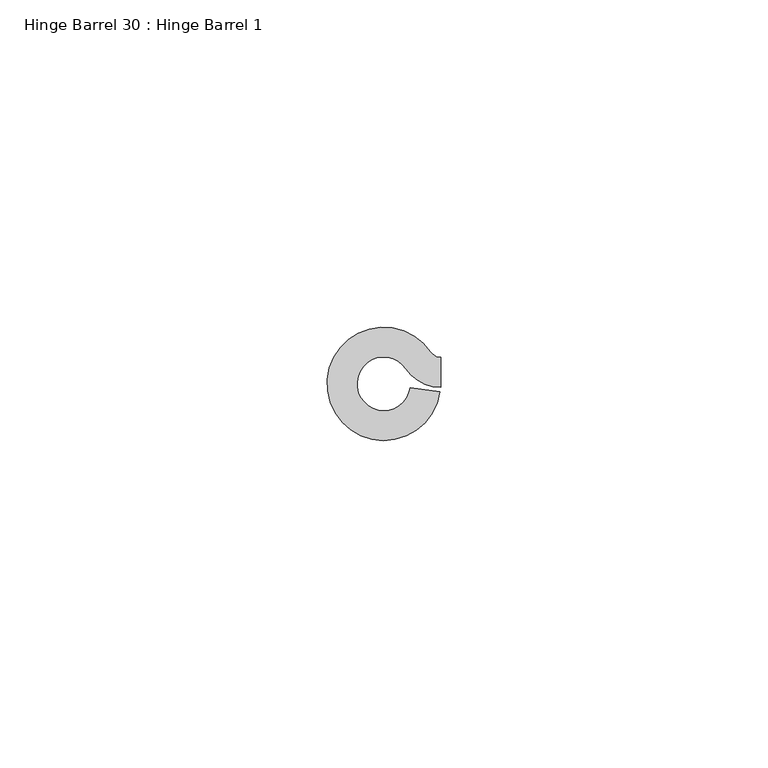
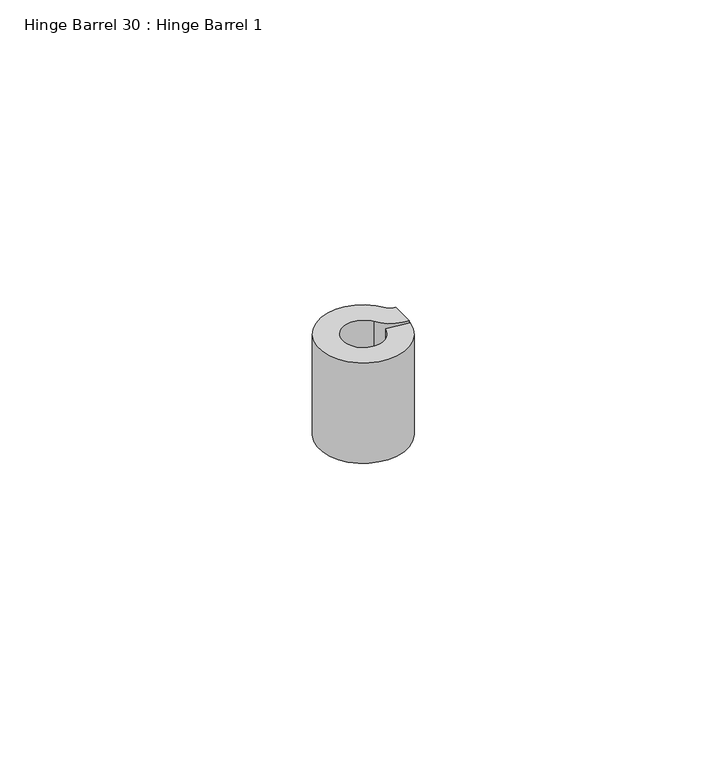
"""IFC4 building model written with IfcOpenShell, lengths in millimetres: proxy geometry, Hinge Barrel 30 : Hinge Barrel 1."""

import ifcopenshell
import ifcopenshell.guid

model = None  # the IFC model being written
_history = None  # IfcOwnerHistory: only IFC2X3 demands one
_inside = {}  # id of a spatial element -> (the spatial element, [elements in it])
_under = {}  # id of a project, library or spatial element -> (it, [spatial elements below it])
_declared = {}  # id of a project -> (the project, [libraries it declares])
_typed = {}  # id of a type object -> (the type object, [elements of that type])
_made_of = {}  # id of a material, layer set ... -> (it, [elements and type objects made of it])


def new_model(schema):
    """Start an empty IFC model of exactly this schema.

    Asked for "IFC4X3", IfcOpenShell would pick the latest addendum, in which some entities
    have other attributes; the version numbers below select the first issue.
    IFC2X3 requires an IfcOwnerHistory on every rooted entity: one is made here for all.
    """
    global model, _history
    if schema == "IFC4X3":
        model = ifcopenshell.file(schema_version=(4, 3, 0, 0))
    else:
        model = ifcopenshell.file(schema=schema)
    _inside.clear()
    _under.clear()
    _declared.clear()
    _typed.clear()
    _made_of.clear()
    _history = None
    if model.schema == "IFC2X3":
        org = make("IfcOrganization", Name="unknown")
        user = make(
            "IfcPersonAndOrganization",
            ThePerson=make("IfcPerson", FamilyName="unknown"),
            TheOrganization=org,
        )
        app = make(
            "IfcApplication",
            ApplicationDeveloper=org,
            Version="unknown",
            ApplicationFullName="unknown",
            ApplicationIdentifier="unknown",
        )
        _history = make(
            "IfcOwnerHistory",
            OwningUser=user,
            OwningApplication=app,
            ChangeAction="ADDED",
            CreationDate=0,
        )
    return model


def make(cls, **values):
    """One entity of the class cls with the attributes given. An attribute that is None is left unset."""
    return model.create_entity(
        cls, **{name: value for name, value in values.items() if value is not None}
    )


def rooted(cls, **values):
    """An entity with a GlobalId (a new one), such as an element, a storey or a relation."""
    return make(cls, GlobalId=ifcopenshell.guid.new(), OwnerHistory=_history, **values)


def si_unit(unit_type, name, prefix=None):
    """IfcSIUnit, for example si_unit("LENGTHUNIT", "METRE", prefix="MILLI")."""
    return make("IfcSIUnit", UnitType=unit_type, Prefix=prefix, Name=name)


def assignment(units):
    """IfcUnitAssignment: the units of a project."""
    return None if units is None else make("IfcUnitAssignment", Units=units)


def point(xyz):
    """IfcCartesianPoint."""
    return None if xyz is None else make("IfcCartesianPoint", Coordinates=xyz)


def direction(xyz):
    """IfcDirection."""
    return None if xyz is None else make("IfcDirection", DirectionRatios=xyz)


def frame(location, z_axis=None, x_axis=None):
    """IfcAxis2Placement3D, a coordinate frame: its origin and axes. An axis left out is left unset."""
    return make(
        "IfcAxis2Placement3D",
        Location=point(location),
        Axis=direction(z_axis),
        RefDirection=direction(x_axis),
    )


def frame_2d(location, x_axis=None):
    """IfcAxis2Placement2D, a coordinate frame in the plane: its origin and x axis."""
    return make(
        "IfcAxis2Placement2D", Location=point(location), RefDirection=direction(x_axis)
    )


def origin():
    """The frame at (0, 0, 0) with its axes left unset."""
    return frame((0.0, 0.0, 0.0))


def place(relative_to, where):
    """IfcLocalPlacement: puts the frame where relative to a parent placement (None: the world)."""
    return make(
        "IfcLocalPlacement", PlacementRelTo=relative_to, RelativePlacement=where
    )


def context(
    kind, dimensions, precision=None, world=None, true_north=None, identifier=None
):
    """IfcGeometricRepresentationContext, for example the 3D "Model" context."""
    return make(
        "IfcGeometricRepresentationContext",
        ContextIdentifier=identifier,
        ContextType=kind,
        CoordinateSpaceDimension=dimensions,
        Precision=precision,
        WorldCoordinateSystem=world,
        TrueNorth=true_north,
    )


def project(units=None, contexts=None):
    """IfcProject with its units and contexts."""
    return rooted(
        "IfcProject",
        Name="project",
        RepresentationContexts=contexts,
        UnitsInContext=assignment(units),
    )


def spatial(cls, under=None, at=None, **own):
    """A site, building, storey or space (cls), placed at a placement, below another one or the project."""
    s = rooted(cls, ObjectPlacement=at, **own)
    if under is not None:
        _under.setdefault(under.id(), (under, []))[1].append(s)
    return s


def polyline(points):
    """IfcPolyline through the points."""
    return make("IfcPolyline", Points=[point(p) for p in points])


def circle_curve(where, radius):
    """IfcCircle in the frame where."""
    return make("IfcCircle", Position=where, Radius=radius)


def trimmed(basis, trim1, trim2, sense, master):
    """IfcTrimmedCurve: the piece of a basis curve between two trims."""
    return make(
        "IfcTrimmedCurve",
        BasisCurve=basis,
        Trim1=trim1,
        Trim2=trim2,
        SenseAgreement=sense,
        MasterRepresentation=master,
    )


def segment(curve, same_sense, transition):
    """IfcCompositeCurveSegment."""
    return make(
        "IfcCompositeCurveSegment",
        Transition=transition,
        SameSense=same_sense,
        ParentCurve=curve,
    )


def composite_curve(segments, self_intersect=None):
    """IfcCompositeCurve: segments joined end to end."""
    return make("IfcCompositeCurve", Segments=segments, SelfIntersect=self_intersect)


def outline(outer, holes=None, kind="AREA"):
    """IfcArbitraryClosedProfileDef: a profile drawn as a closed curve; with holes, ...WithVoids."""
    if holes is None:
        return make("IfcArbitraryClosedProfileDef", ProfileType=kind, OuterCurve=outer)
    return make(
        "IfcArbitraryProfileDefWithVoids",
        ProfileType=kind,
        OuterCurve=outer,
        InnerCurves=holes,
    )


def extrude(swept, where, along, depth):
    """IfcExtrudedAreaSolid: the profile swept, set in the frame where, extruded along a direction by depth."""
    return make(
        "IfcExtrudedAreaSolid",
        SweptArea=swept,
        Position=where,
        ExtrudedDirection=direction(along),
        Depth=depth,
    )


def shape(context_of_items, identifier, shape_type, items):
    """IfcShapeRepresentation: the items that make up one representation, for example the "Body"."""
    return make(
        "IfcShapeRepresentation",
        ContextOfItems=context_of_items,
        RepresentationIdentifier=identifier,
        RepresentationType=shape_type,
        Items=items,
    )


def source(mapping_origin, context_of_items, identifier, shape_type, items):
    """IfcRepresentationMap: a shape defined once, which mapped items show again and again."""
    return make(
        "IfcRepresentationMap",
        MappingOrigin=mapping_origin,
        MappedRepresentation=shape(context_of_items, identifier, shape_type, items),
    )


def transform(
    local_origin,
    x_axis=None,
    y_axis=None,
    z_axis=None,
    scale=None,
    scale2=None,
    scale3=None,
    uniform=True,
):
    """IfcCartesianTransformationOperator3D, or its non-uniform kind. x_axis, y_axis, z_axis: its Axis1, 2, 3."""
    if uniform:
        return make(
            "IfcCartesianTransformationOperator3D",
            Axis1=direction(x_axis),
            Axis2=direction(y_axis),
            LocalOrigin=point(local_origin),
            Scale=scale,
            Axis3=direction(z_axis),
        )
    return make(
        "IfcCartesianTransformationOperator3DnonUniform",
        Axis1=direction(x_axis),
        Axis2=direction(y_axis),
        LocalOrigin=point(local_origin),
        Scale=scale,
        Axis3=direction(z_axis),
        Scale2=scale2,
        Scale3=scale3,
    )


def mapped(mapping_source, mapping_target):
    """IfcMappedItem: shows the shape of a source again, moved by a transform."""
    return make(
        "IfcMappedItem", MappingSource=mapping_source, MappingTarget=mapping_target
    )


def made_of(thing, what):
    """Note that an element or type object is made of a material, layer set ...; save() writes the relation."""
    if what is not None:
        _made_of.setdefault(what.id(), (what, []))[1].append(thing)
    return thing


def element(
    cls,
    number,
    at=None,
    inside=None,
    cuts=None,
    type_object=None,
    material=None,
    context=None,
    identifier="Body",
    shape_type=None,
    held_by="IfcProductDefinitionShape",
    body=None,
    shapes=None,
    **own,
):
    """One element of the class cls, such as IfcWall. Its Tag is "e" and its number.

    at: its placement. inside: the storey or other place that contains it. cuts: it is an
    opening in that element (IfcRelVoidsElement). A single representation is given by context,
    identifier, shape_type and body (its items); several are given by shapes. held_by: the class
    of the entity that holds the representations. save() writes the other relations.
    """
    e = rooted(cls, Tag="e%d" % number, ObjectPlacement=at, **own)
    if body is not None:
        shapes = [shape(context, identifier, shape_type, body)]
    if shapes is not None:
        e.Representation = make(held_by, Representations=shapes)
    if inside is not None:
        _inside.setdefault(inside.id(), (inside, []))[1].append(e)
    if cuts is not None:
        rooted(
            "IfcRelVoidsElement", RelatingBuildingElement=cuts, RelatedOpeningElement=e
        )
    if type_object is not None:
        _typed.setdefault(type_object.id(), (type_object, []))[1].append(e)
    return made_of(e, material)


def aggregate(whole, parts):
    """IfcRelAggregates: a whole, such as a stair, and the parts it consists of."""
    return rooted("IfcRelAggregates", RelatingObject=whole, RelatedObjects=parts)


def save(model, path):
    """Write the relations noted so far, then the file.

    IfcRelAggregates (storeys below a building ...), IfcRelContainedInSpatialStructure (elements
    in a storey), IfcRelDefinesByType, IfcRelAssociatesMaterial and IfcRelDeclares: one each for
    every whole, place, type object, material and project.
    """
    for whole, parts in _under.values():
        aggregate(whole, parts)
    for where, things in _inside.values():
        rooted(
            "IfcRelContainedInSpatialStructure",
            RelatedElements=things,
            RelatingStructure=where,
        )
    for kind, things in _typed.values():
        rooted("IfcRelDefinesByType", RelatedObjects=things, RelatingType=kind)
    for what, things in _made_of.values():
        rooted("IfcRelAssociatesMaterial", RelatedObjects=things, RelatingMaterial=what)
    for by, libraries in _declared.values():
        rooted("IfcRelDeclares", RelatingContext=by, RelatedDefinitions=libraries)
    model.write(path)


def hinge_barrel_30_hinge_barrel_1_18e6ea9c(model_context):
    return source(origin(), model_context, "Body", "SweptSolid", [
        extrude(outline(composite_curve([segment(trimmed(circle_curve(frame_2d((587319.1320739, -531776.6049841)), 4.0894), [point((587322.5194669, -531774.3139665))], [point((587323.1821338, -531777.1708529))], True, "CARTESIAN"), True, "CONTINUOUS"), segment(polyline([(587323.1821338, -531777.1708529), (587327.7022899, -531777.8024028)]), True, "CONTINUOUS"), segment(trimmed(circle_curve(frame_2d((587319.1320739, -531776.6049841)), 8.6534625), [point((587327.7022899, -531777.8024028))], [point((587326.3000393, -531771.7570273))], False, "CARTESIAN"), True, "CONTINUOUS"), segment(trimmed(circle_curve(frame_2d((587327.8245257, -531770.7259615)), 1.8404226), [point((587326.3000393, -531771.7570273))], [point((587327.8245257, -531772.5663841))], True, "CARTESIAN"), True, "CONTINUOUS"), segment(polyline([(587327.8245257, -531772.5663841), (587327.8245257, -531777.1304466)]), True, "CONTINUOUS"), segment(trimmed(circle_curve(frame_2d((587327.8245257, -531770.7259615)), 6.4044851), [point((587327.8245257, -531777.1304466))], [point((587322.5194669, -531774.3139665))], False, "CARTESIAN"), True, "CONTINUOUS")], self_intersect=False)), frame((0.0, 0.0, 1250.95), z_axis=(0.0, 0.0, 1.0), x_axis=(1.0, 0.0, 0.0)), (0.0, 0.0, 1.0), 20.8359375),
    ])


if __name__ == "__main__":
    model = new_model("IFC4")
    model_context = context("Model", 3, world=origin())
    ifc_project = project(units=[si_unit("LENGTHUNIT", "METRE", prefix="MILLI")], contexts=[model_context])
    site = spatial("IfcSite", under=ifc_project)
    building = spatial("IfcBuilding", under=site)
    placement = place(None, origin())
    hinge_barrel_30_hinge_barrel_1_shape = hinge_barrel_30_hinge_barrel_1_18e6ea9c(model_context)
    element("IfcBuildingElementProxy", 1, Name="Hinge Barrel 30 : Hinge Barrel 1", ObjectType="Hinge Barrel 30 : Hinge Barrel 1", at=placement, inside=building, context=model_context, shape_type="MappedRepresentation", body=[
        mapped(hinge_barrel_30_hinge_barrel_1_shape, transform((0.0, 0.0, 0.0), x_axis=(1.0, 0.0, 0.0), y_axis=(0.0, 1.0, 0.0), z_axis=(0.0, 0.0, 1.0))),
    ])
    save(model, "model.ifc")

# Revit data of these elements
# Element 1 (IfcBuildingElementProxy, "Hinge Barrel 30 : Hinge Barrel 1")
#   Materials on its faces: "6\"X6\" WELD-ON STL BUTT HINGE"
# Materials
#   "6\"X6\" WELD-ON STL BUTT HINGE": class "Metal", colour RGB 189 187 185, transparency 0, Description = "Carbon steel", Cost = 0
